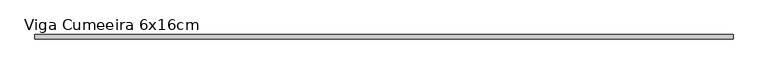
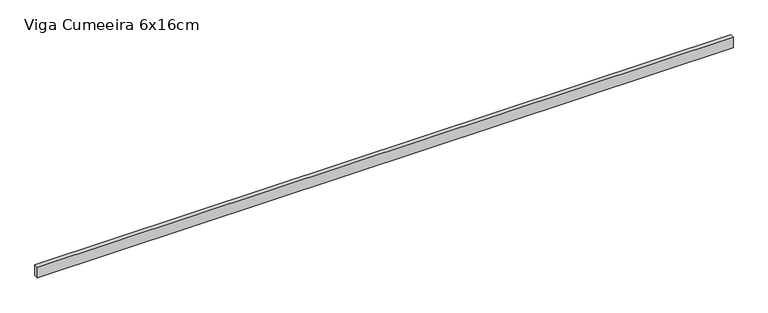
"""IFC4 building model written with IfcOpenShell, lengths in millimetres: beam geometry, Madeira de lei : Viga Cumeeira 6x16cm."""

from ifc_helpers import new_model, si_unit, frame, origin, place, context, project, spatial, polyline, outline, extrude, source, transform, mapped, element, save


def viga_cumeeira_6x16cm_5eb8e513(model_context):
    return source(origin(), model_context, "Body", "SweptSolid", [
        extrude(outline(polyline([(4969.5, 30.0), (4969.5, -30.0), (-4969.5, -30.0), (-4969.5, 30.0), (4969.5, 30.0)])), frame((0.0, 0.0, -80.0), z_axis=(0.0, 0.0, 1.0), x_axis=(1.0, 0.0, 0.0)), (0.0, 0.0, 1.0), 160.0),
    ])


if __name__ == "__main__":
    model = new_model("IFC4")
    model_context = context("Model", 3, world=origin())
    ifc_project = project(units=[si_unit("LENGTHUNIT", "METRE", prefix="MILLI")], contexts=[model_context])
    site = spatial("IfcSite", under=ifc_project)
    building = spatial("IfcBuilding", under=site)
    placement = place(None, origin())
    viga_cumeeira_6x16cm_shape = viga_cumeeira_6x16cm_5eb8e513(model_context)
    element("IfcBeam", 1, ObjectType="Madeira de lei : Viga Cumeeira 6x16cm", at=placement, inside=building, context=model_context, shape_type="MappedRepresentation", body=[
        mapped(viga_cumeeira_6x16cm_shape, transform((0.0, 0.0, 0.0), x_axis=(1.0, 0.0, 0.0), y_axis=(0.0, 1.0, 0.0), z_axis=(0.0, 0.0, 1.0))),
    ])
    save(model, "model.ifc")

# Revit data of these elements
# Type "Madeira de lei : Viga Cumeeira 6x16cm"
#   A = 0.02 m²
#   Length [instance default] = 1.524 m
#   b = 0.06 m
#   d = 0.16 m
#   Structural Material [instance default] = none
#   Assembly Code = ""
# Element 1 (IfcBeam, "Madeira de lei : Viga Cumeeira 6x16cm")
#   Structural Material = .MADEIRAMENTO
#   Materials on its faces: ".MADEIRAMENTO"
# Materials
#   ".MADEIRAMENTO": class ".CC_MADEIRAS", colour RGB 212 179 113, transparency 0, Cost = 0
